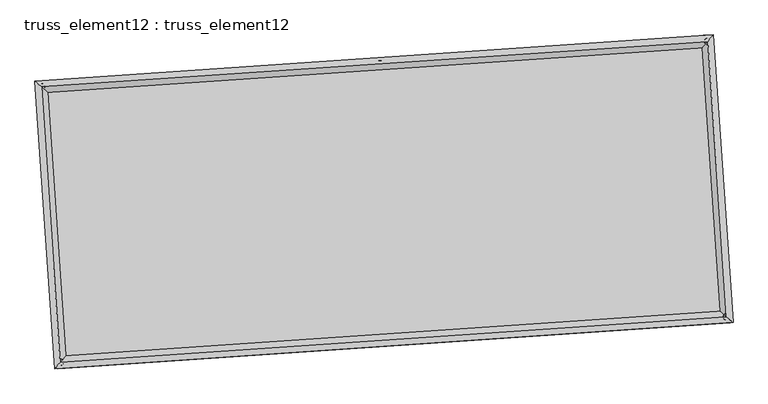
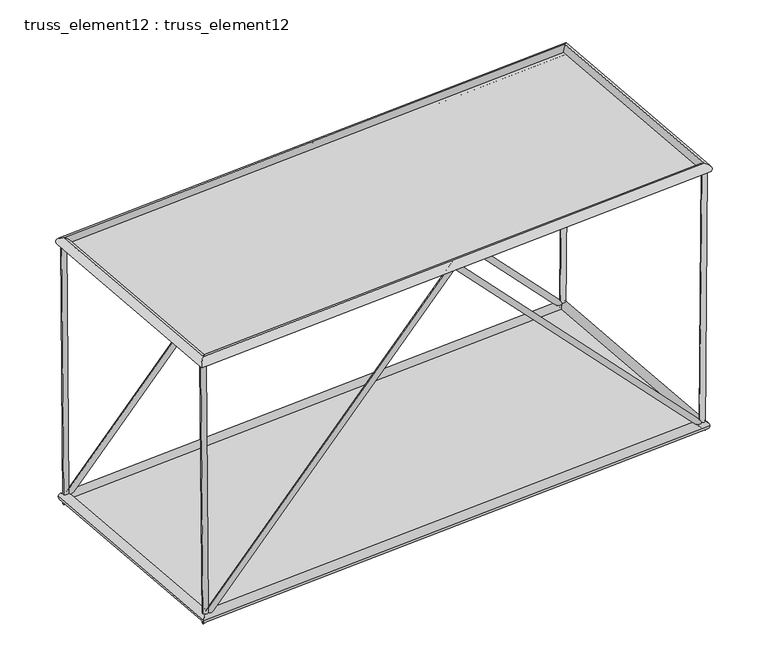
"""IFC4 building model written with IfcOpenShell, lengths in millimetres: plate geometry, truss_element12 : truss_element12."""

from ifc_helpers import new_model, si_unit, frame, origin, origin_with_axes, place, context, project, spatial, polyline, circle_curve, ellipse_curve, outline, extrude, source, transform, mapped, element, save
from ifc_brep_helpers import plane_surface, cylinder_surface, advanced_brep


def truss_element12_truss_element12_78f2e21b(model_context):
    return source(origin(), model_context, "Body", "SolidModel", [
        advanced_brep(
        [(-3708.7284358, 2273.2383309, 5000.2453052), (-3807.8279627, 2259.8773169, 4999.3694838), (-3666.0177363, 2276.1506111, 123.0852672), (-3762.9691466, 2262.936069, -123.0852672), (1063.3506953, 2598.6282664, 5071.9331177), (1063.8044049, 2592.0554092, 4927.6880571), (5793.4386673, 2921.1549845, 123.0904417), (5891.3223097, 2921.225504, -123.0904417), (5835.4352687, 2924.0185731, 5000.2443705), (5935.4313303, 2924.2331304, 4999.3831901)],
        [
            (0, 1, circle_curve(frame((-3758.2781993, 2266.5578239, 4999.8073945), z_axis=(-0.00875695156738304, -0.000597103239090544, 0.9999614788915464), x_axis=(-0.13361022272283757, 0.9910337905255439, -0.0005782910393320115)), 50.0)),
            (1, 0, circle_curve(frame((-3758.2781993, 2266.5578239, 4999.8073945), z_axis=(-0.00875695156738304, -0.000597103239090544, 0.9999614788915464), x_axis=(-0.13361022272283757, 0.9910337905255439, -0.0005782910393320115)), 50.0)),
            (0, 2),
            (2, 3, ellipse_curve(frame((-3714.4934414, 2269.54334, 0.0), z_axis=(-0.9274161456323371, -0.06323698153185056, 0.36864668313603527), x_axis=(0.3677926747828987, 0.02507838438259889, 0.929569590193655)), 132.6993561, 50.0)),
            (3, 1),
            (3, 2, ellipse_curve(frame((-3714.4934414, 2269.54334, 0.0), z_axis=(-0.9274161456323371, -0.06323698153185056, 0.36864668313603527), x_axis=(0.3677926747828987, 0.02507838438259889, 0.929569590193655)), 132.6993561, 50.0)),
            (2, 4),
            (4, 5, ellipse_curve(frame((1063.5775501, 2595.3418378, 4999.8105874), z_axis=(-0.9976833953446987, -0.06802823817891356, -3.8258939129589834e-05), x_axis=(3.817030832084858e-05, 2.602688225433117e-06, -0.9999999992681268)), 72.2795775, 50.0)),
            (5, 3),
            (5, 4, ellipse_curve(frame((1063.5775501, 2595.3418378, 4999.8105874), z_axis=(-0.9976833953446987, -0.06802823817891356, -3.8258939129589834e-05), x_axis=(3.817030832084858e-05, 2.602688225433117e-06, -0.9999999992681268)), 72.2795775, 50.0)),
            (4, 6),
            (6, 7, ellipse_curve(frame((5842.3804885, 2921.1902443, 0.0), z_axis=(-0.9273750844968214, -0.06323418172910764, -0.36875044530897005), x_axis=(-0.3678961965799763, -0.025085443140418415, 0.9295284337148791)), 132.7108104, 50.0)),
            (7, 5),
            (7, 6, ellipse_curve(frame((5842.3804885, 2921.1902443, 0.0), z_axis=(-0.9273750844968214, -0.06323418172910764, -0.36875044530897005), x_axis=(-0.3678961965799763, -0.025085443140418415, 0.9295284337148791)), 132.7108104, 50.0)),
            (8, 9, circle_curve(frame((5885.4332995, 2924.1258518, 4999.8137803), z_axis=(0.008610562197328536, 0.0005871215044245873, 0.999962756059937), x_axis=(-0.0021505497839294303, 0.9999975258982473, -0.0005686237869435077)), 50.0)),
            (9, 8, circle_curve(frame((5885.4332995, 2924.1258518, 4999.8137803), z_axis=(0.008610562197328536, 0.0005871215044245873, 0.999962756059937), x_axis=(-0.0021505497839294303, 0.9999975258982473, -0.0005686237869435077)), 50.0)),
            (6, 8),
            (9, 7),
        ],
        [
            plane_surface(frame((-3758.2781993, 2316.5578149, 4999.8372508), z_axis=(-0.00875695156738239, -0.0005971032390901988, 0.9999614788915465), x_axis=(0.9999616571645369, -5.229004639950574e-06, 0.008756950006194586))),
            cylinder_surface(frame((-3758.2781993, 2266.5578239, 4999.8073945), z_axis=(-0.00875695156738304, -0.000597103239090544, 0.9999614788915464), x_axis=(-0.13361022272283757, 0.9910337905255439, -0.0005782910393320115)), 50.0),
            cylinder_surface(frame((-3714.4934414, 2269.54334, 0.0), z_axis=(-0.6901282375994741, -0.047057221098874086, -0.722155546686651), x_axis=(-0.02041146399559655, 0.9987523835743873, -0.04557464692168603)), 50.0),
            cylinder_surface(frame((1063.5775501, 2595.3418378, 4999.8105874), z_axis=(-0.6901833653788336, -0.04706098005258826, 0.7221026148068135), x_axis=(-0.11534591312680834, 0.9922791643677564, -0.04557828744665373)), 50.0),
            plane_surface(frame((5885.4332995, 2874.1258604, 4999.8431375), z_axis=(0.008610562197328036, 0.0005871215044280536, 0.9999627560599371), x_axis=(0.999962928422172, -5.055633652162332e-06, -0.008610560713137268))),
            cylinder_surface(frame((5842.3804885, 2921.1902443, 0.0), z_axis=(-0.008610562197328536, -0.0005871215044245873, -0.999962756059937), x_axis=(-0.0021505497839294303, 0.9999975258982473, -0.0005686237869435077)), 50.0),
        ],
        [
            (0, [[1, 2]]),
            (1, [[-1, 3, 4, 5]]),
            (1, [[-2, -5, 6, -3]]),
            (2, [[-4, 7, 8, 9]]),
            (2, [[-6, -9, 10, -7]]),
            (3, [[-8, 11, 12, 13]]),
            (3, [[-10, -13, 14, -11]]),
            (4, [[15, 16]]),
            (5, [[-12, 17, -16, 18]]),
            (5, [[-14, -18, -15, -17]]),
        ],
    ),
        advanced_brep(
        [(-3436.6154829, -1717.4952534, 5000.2453052), (-3535.7150098, -1730.8562674, 4999.3694838), (-3393.9047834, -1714.5829732, 123.0852672), (-3490.8561936, -1727.7975153, -123.0852672), (1335.4636482, -1392.1053179, 5071.9331177), (1335.9173578, -1398.6781751, 4927.6880571), (6065.5516202, -1069.5785998, 123.0904417), (6163.4352626, -1069.5080803, -123.0904417), (6107.5482216, -1066.7150112, 5000.2443705), (6207.5442832, -1066.5004539, 4999.3831901)],
        [
            (0, 1, circle_curve(frame((-3486.1652463, -1724.1757604, 4999.8073945), z_axis=(-0.008756951567383037, -0.000597103239090551, 0.9999614788915463), x_axis=(-0.13361022272283762, 0.9910337905255439, -0.0005782910393320047)), 50.0)),
            (1, 0, circle_curve(frame((-3486.1652463, -1724.1757604, 4999.8073945), z_axis=(-0.008756951567383037, -0.000597103239090551, 0.9999614788915463), x_axis=(-0.13361022272283762, 0.9910337905255439, -0.0005782910393320047)), 50.0)),
            (0, 2),
            (2, 3, ellipse_curve(frame((-3442.3804885, -1721.1902443, 0.0), z_axis=(-0.927416145632337, -0.06323698153185059, 0.36864668313603505), x_axis=(0.3677926747828984, 0.02507838438259887, 0.9295695901936551)), 132.6993561, 50.0)),
            (3, 1),
            (3, 2, ellipse_curve(frame((-3442.3804885, -1721.1902443, 0.0), z_axis=(-0.927416145632337, -0.06323698153185059, 0.36864668313603505), x_axis=(0.3677926747828984, 0.02507838438259887, 0.9295695901936551)), 132.6993561, 50.0)),
            (2, 4),
            (4, 5, ellipse_curve(frame((1335.690503, -1395.3917465, 4999.8105874), z_axis=(-0.9976833953446987, -0.0680282381789137, -3.82589391300713e-05), x_axis=(3.8170308321309824e-05, 2.602688225586861e-06, -0.9999999992681268)), 72.2795775, 50.0)),
            (5, 3),
            (5, 4, ellipse_curve(frame((1335.690503, -1395.3917465, 4999.8105874), z_axis=(-0.9976833953446987, -0.0680282381789137, -3.82589391300713e-05), x_axis=(3.8170308321309824e-05, 2.602688225586861e-06, -0.9999999992681268)), 72.2795775, 50.0)),
            (4, 6),
            (6, 7, ellipse_curve(frame((6114.4934414, -1069.54334, 0.0), z_axis=(-0.927375084496821, -0.06323418172910777, -0.36875044530897083), x_axis=(-0.3678961965799771, -0.02508544314041859, 0.9295284337148788)), 132.7108104, 50.0)),
            (7, 5),
            (7, 6, ellipse_curve(frame((6114.4934414, -1069.54334, 0.0), z_axis=(-0.927375084496821, -0.06323418172910777, -0.36875044530897083), x_axis=(-0.3678961965799771, -0.02508544314041859, 0.9295284337148788)), 132.7108104, 50.0)),
            (8, 9, circle_curve(frame((6157.5462524, -1066.6077325, 4999.8137803), z_axis=(0.00861056219732793, 0.0005871215044244897, 0.999962756059937), x_axis=(-0.0021505497839295275, 0.9999975258982473, -0.0005686237869434106)), 50.0)),
            (9, 8, circle_curve(frame((6157.5462524, -1066.6077325, 4999.8137803), z_axis=(0.00861056219732793, 0.0005871215044244897, 0.999962756059937), x_axis=(-0.0021505497839295275, 0.9999975258982473, -0.0005686237869434106)), 50.0)),
            (6, 8),
            (9, 7),
        ],
        [
            plane_surface(frame((-3486.1652463, -1674.1757694, 4999.8372508), z_axis=(-0.00875695156738239, -0.0005971032390902037, 0.9999614788915465), x_axis=(0.9999616571645369, -5.229004639950574e-06, 0.008756950006194586))),
            cylinder_surface(frame((-3486.1652463, -1724.1757604, 4999.8073945), z_axis=(-0.008756951567383037, -0.000597103239090551, 0.9999614788915463), x_axis=(-0.13361022272283762, 0.9910337905255439, -0.0005782910393320047)), 50.0),
            cylinder_surface(frame((-3442.3804885, -1721.1902443, 0.0), z_axis=(-0.6901282375994737, -0.04705722109887407, -0.7221555466866512), x_axis=(-0.020411463995596478, 0.9987523835743873, -0.045574646921686085)), 50.0),
            cylinder_surface(frame((1335.690503, -1395.3917465, 4999.8105874), z_axis=(-0.6901833653788342, -0.04706098005258848, 0.722102614806813), x_axis=(-0.11534591312680864, 0.9922791643677564, -0.045578287446653855)), 50.0),
            plane_surface(frame((6157.5462524, -1116.6077239, 4999.8431375), z_axis=(0.008610562197328036, 0.0005871215044280584, 0.9999627560599371), x_axis=(0.999962928422172, -5.055633651718243e-06, -0.008610560713137268))),
            cylinder_surface(frame((6114.4934414, -1069.54334, 0.0), z_axis=(-0.00861056219732793, -0.0005871215044244897, -0.999962756059937), x_axis=(-0.0021505497839295275, 0.9999975258982473, -0.0005686237869434106)), 50.0),
        ],
        [
            (0, [[1, 2]]),
            (1, [[-1, 3, 4, 5]]),
            (1, [[-2, -5, 6, -3]]),
            (2, [[-4, 7, 8, 9]]),
            (2, [[-6, -9, 10, -7]]),
            (3, [[-8, 11, 12, 13]]),
            (3, [[-10, -13, 14, -11]]),
            (4, [[15, 16]]),
            (5, [[-12, 17, -16, 18]]),
            (5, [[-14, -18, -15, -17]]),
        ],
    ),
        advanced_brep(
        [(-3486.1635638, -1724.1738957, 4909.8073945), (-3486.1669288, -1724.1776252, 5089.8073944), (-3758.2801193, 2266.559443, 5089.8073944), (-3758.2762792, 2266.5562047, 4909.8073945), (5885.4348634, 2924.1277085, 5089.8137803), (5885.4317356, 2924.1239951, 4909.8137803), (6157.5480538, -1066.6093598, 5089.8137803), (6157.544451, -1066.6061053, 4909.8137803)],
        [
            (0, 1, ellipse_curve(frame((-3486.1652463, -1724.1757604, 4999.8073945), z_axis=(-0.7535719234053031, 0.6573654662780922, -4.6714499764974463e-07), x_axis=(-0.6573654662779277, -0.7535719234054468, -4.6714499764974553e-07)), 127.2792206, 90.0)),
            (1, 2),
            (2, 3, ellipse_curve(frame((-3758.2781993, 2266.5578239, 4999.8073945), z_axis=(-0.6573654662779277, -0.7535719234054467, -4.671449976497484e-07), x_axis=(0.7535719234053031, -0.6573654662780923, 4.6714499764974744e-07)), 127.2792206, 90.0)),
            (3, 0),
            (1, 0, ellipse_curve(frame((-3486.1652463, -1724.1757604, 4999.8073945), z_axis=(-0.7535719234053031, 0.6573654662780922, -4.6714499764974463e-07), x_axis=(-0.6573654662779277, -0.7535719234054468, -4.6714499764974553e-07)), 127.2792206, 90.0)),
            (3, 2, ellipse_curve(frame((-3758.2781993, 2266.5578239, 4999.8073945), z_axis=(-0.6573654662779277, -0.7535719234054467, -4.671449976497484e-07), x_axis=(0.7535719234053031, -0.6573654662780923, 4.6714499764974744e-07)), 127.2792206, 90.0)),
            (2, 4),
            (4, 5, ellipse_curve(frame((5885.4332995, 2924.1258518, 4999.8137803), z_axis=(-0.7535719234053033, 0.657365466278092, -4.671449976497499e-07), x_axis=(-0.6573654662779277, -0.7535719234054468, -4.6714499764974617e-07)), 127.2792206, 90.0)),
            (5, 3),
            (5, 4, ellipse_curve(frame((5885.4332995, 2924.1258518, 4999.8137803), z_axis=(-0.7535719234053033, 0.657365466278092, -4.671449976497499e-07), x_axis=(-0.6573654662779277, -0.7535719234054468, -4.6714499764974617e-07)), 127.2792206, 90.0)),
            (4, 6),
            (6, 7, ellipse_curve(frame((6157.5462524, -1066.6077325, 4999.8137803), z_axis=(0.6573654662779277, 0.7535719234054468, 4.671449976497433e-07), x_axis=(-0.7535719234053033, 0.657365466278092, -4.67144997649747e-07)), 127.2792206, 90.0)),
            (7, 5),
            (7, 6, ellipse_curve(frame((6157.5462524, -1066.6077325, 4999.8137803), z_axis=(0.6573654662779277, 0.7535719234054468, 4.671449976497433e-07), x_axis=(-0.7535719234053033, 0.657365466278092, -4.67144997649747e-07)), 127.2792206, 90.0)),
            (6, 1),
            (0, 7),
        ],
        [
            cylinder_surface(frame((-3486.1652463, -1724.1757604, 4999.8073945), z_axis=(0.06802823822869847, -0.9976833960748769, 0.0), x_axis=(-0.9976833958741261, -0.06802823821501004, -2.0060750292057037e-05)), 90.0),
            cylinder_surface(frame((-3758.2781993, 2266.5578239, 4999.8073945), z_axis=(-0.997683396074659, -0.06802823822868682, -6.606427912710213e-07), x_axis=(-0.06802823820311313, 0.9976833958880024, -1.9400107500910345e-05)), 90.0),
            cylinder_surface(frame((5885.4332995, 2924.1258518, 4999.8137803), z_axis=(-0.06802823822869869, 0.9976833960748768, 0.0), x_axis=(0.9976833958996998, 0.06802823821675404, -1.8739464709763642e-05)), 90.0),
            cylinder_surface(frame((6157.5462524, -1066.6077325, 4999.8137803), z_axis=(0.997683396074659, 0.06802823822868669, 6.606427912710173e-07), x_axis=(0.06802823822868669, -0.9976833958862587, -1.9400107500910338e-05)), 90.0),
        ],
        [
            (0, [[1, 2, 3, 4]]),
            (0, [[5, -4, 6, -2]]),
            (1, [[-3, 7, 8, 9]]),
            (1, [[-6, -9, 10, -7]]),
            (2, [[-8, 11, 12, 13]]),
            (2, [[-10, -13, 14, -11]]),
            (3, [[-12, 15, -1, 16]]),
            (3, [[-14, -16, -5, -15]]),
        ],
    ),
        advanced_brep(
        [(-3358.7115243, -1625.2761972, 0.0), (-3526.0494527, -1817.1042913, 0.0), (-3810.4074885, 2353.2123043, 0.0), (-3618.5793943, 2185.8743758, 0.0), (5926.0494527, 3017.1042913, 0.0), (5758.7115243, 2825.2761972, 0.0), (6210.4074885, -1153.2123043, 0.0), (6018.5793943, -985.8743758, 0.0)],
        [
            (0, 1, ellipse_curve(frame((-3442.3804885, -1721.1902443, 0.0), z_axis=(-0.7535719234054573, 0.6573654662780813, 0.0), x_axis=(-0.6573654662780812, -0.7535719234054575, 0.0)), 127.2792206, 90.0)),
            (1, 2),
            (2, 3, ellipse_curve(frame((-3714.4934414, 2269.54334, 0.0), z_axis=(-0.6573654662780815, -0.7535719234054575, 0.0), x_axis=(0.7535719234054576, -0.6573654662780811, 0.0)), 127.2792206, 90.0)),
            (3, 0),
            (1, 0, ellipse_curve(frame((-3442.3804885, -1721.1902443, 0.0), z_axis=(-0.7535719234054573, 0.6573654662780813, 0.0), x_axis=(-0.6573654662780812, -0.7535719234054575, 0.0)), 127.2792206, 90.0)),
            (3, 2, ellipse_curve(frame((-3714.4934414, 2269.54334, 0.0), z_axis=(-0.6573654662780815, -0.7535719234054575, 0.0), x_axis=(0.7535719234054576, -0.6573654662780811, 0.0)), 127.2792206, 90.0)),
            (2, 4),
            (4, 5, ellipse_curve(frame((5842.3804885, 2921.1902443, 0.0), z_axis=(-0.7535719234054573, 0.6573654662780815, 0.0), x_axis=(-0.6573654662780816, -0.7535719234054573, 0.0)), 127.2792206, 90.0)),
            (5, 3),
            (5, 4, ellipse_curve(frame((5842.3804885, 2921.1902443, 0.0), z_axis=(-0.7535719234054573, 0.6573654662780815, 0.0), x_axis=(-0.6573654662780816, -0.7535719234054573, 0.0)), 127.2792206, 90.0)),
            (4, 6),
            (6, 7, ellipse_curve(frame((6114.4934414, -1069.54334, 0.0), z_axis=(0.6573654662780817, 0.7535719234054572, 0.0), x_axis=(-0.7535719234054572, 0.6573654662780817, 0.0)), 127.2792206, 90.0)),
            (7, 5),
            (7, 6, ellipse_curve(frame((6114.4934414, -1069.54334, 0.0), z_axis=(0.6573654662780817, 0.7535719234054572, 0.0), x_axis=(-0.7535719234054572, 0.6573654662780817, 0.0)), 127.2792206, 90.0)),
            (6, 1),
            (0, 7),
        ],
        [
            cylinder_surface(frame((-3442.3804885, -1721.1902443, 0.0), z_axis=(0.068028238228699, -0.9976833960748768, 0.0), x_axis=(-0.9976833960748768, -0.068028238228699, 0.0)), 90.0),
            cylinder_surface(frame((-3714.4934414, 2269.54334, 0.0), z_axis=(-0.9976833960748765, -0.06802823822870196, 0.0), x_axis=(-0.06802823822870196, 0.9976833960748765, 0.0)), 90.0),
            cylinder_surface(frame((5842.3804885, 2921.1902443, 0.0), z_axis=(-0.06802823822869876, 0.9976833960748768, 0.0), x_axis=(0.9976833960748768, 0.06802823822869876, 0.0)), 90.0),
            cylinder_surface(frame((6114.4934414, -1069.54334, 0.0), z_axis=(0.9976833960748767, 0.0680282382287017, 0.0), x_axis=(0.0680282382287017, -0.9976833960748767, 0.0)), 90.0),
        ],
        [
            (0, [[1, 2, 3, 4]]),
            (0, [[5, -4, 6, -2]]),
            (1, [[-3, 7, 8, 9]]),
            (1, [[-6, -9, 10, -7]]),
            (2, [[-8, 11, 12, 13]]),
            (2, [[-10, -13, 14, -11]]),
            (3, [[-12, 15, -1, 16]]),
            (3, [[-14, -16, -5, -15]]),
        ],
    ),
        extrude(outline(polyline([(-3442.3804885, -1721.1902443), (-3714.4934414, 2269.54334), (5842.3804885, 2921.1902443), (6114.4934414, -1069.54334), (-3442.3804885, -1721.1902443)])), origin_with_axes(), (0.0, 0.0, 1.0), 20.0),
        extrude(outline(polyline([(-2000.0, 4833.0520166), (2000.0, 4833.0520167), (2000.0, -4833.0520166), (-2000.0, -4833.0520166), (-2000.0, 4833.0520166)])), frame((1199.6340266, 599.9750457, 4999.8105874), z_axis=(-6.591123435876566e-07, -4.494236518865731e-08, 0.999999999999782), x_axis=(-0.06802823822869858, 0.9976833960748768, 0.0)), (0.0, 0.0, 1.0), 20.0),
    ])


if __name__ == "__main__":
    model = new_model("IFC4")
    model_context = context("Model", 3, world=origin())
    ifc_project = project(units=[si_unit("LENGTHUNIT", "METRE", prefix="MILLI")], contexts=[model_context])
    site = spatial("IfcSite", under=ifc_project)
    building = spatial("IfcBuilding", under=site)
    placement = place(None, origin())
    truss_element12_truss_element12_shape = truss_element12_truss_element12_78f2e21b(model_context)
    element("IfcPlate", 1, ObjectType="truss_element12 : truss_element12", at=placement, inside=building, context=model_context, shape_type="MappedRepresentation", body=[
        mapped(truss_element12_truss_element12_shape, transform((0.0, 0.0, 0.0), x_axis=(1.0, 0.0, 0.0), y_axis=(0.0, 1.0, 0.0), z_axis=(0.0, 0.0, 1.0))),
    ])
    save(model, "model.ifc")

# Revit data of these elements
# Type "truss_element12 : truss_element12"
#   steellbar1 = 90 mm
#   steelbar2 = 50 mm
#   offset1 = 5000 mm
#   M = Default Roof
# Element 1 (IfcPlate, "truss_element12 : truss_element12")
#   Materials on its faces: "Default Roof"
# Materials
#   "Default Roof": class "Miscellaneous", colour RGB 0 127 0, transparency 0, Comments = "Rendering appearance not upgraded Rendering appearance not upgraded ", Cost = 0
